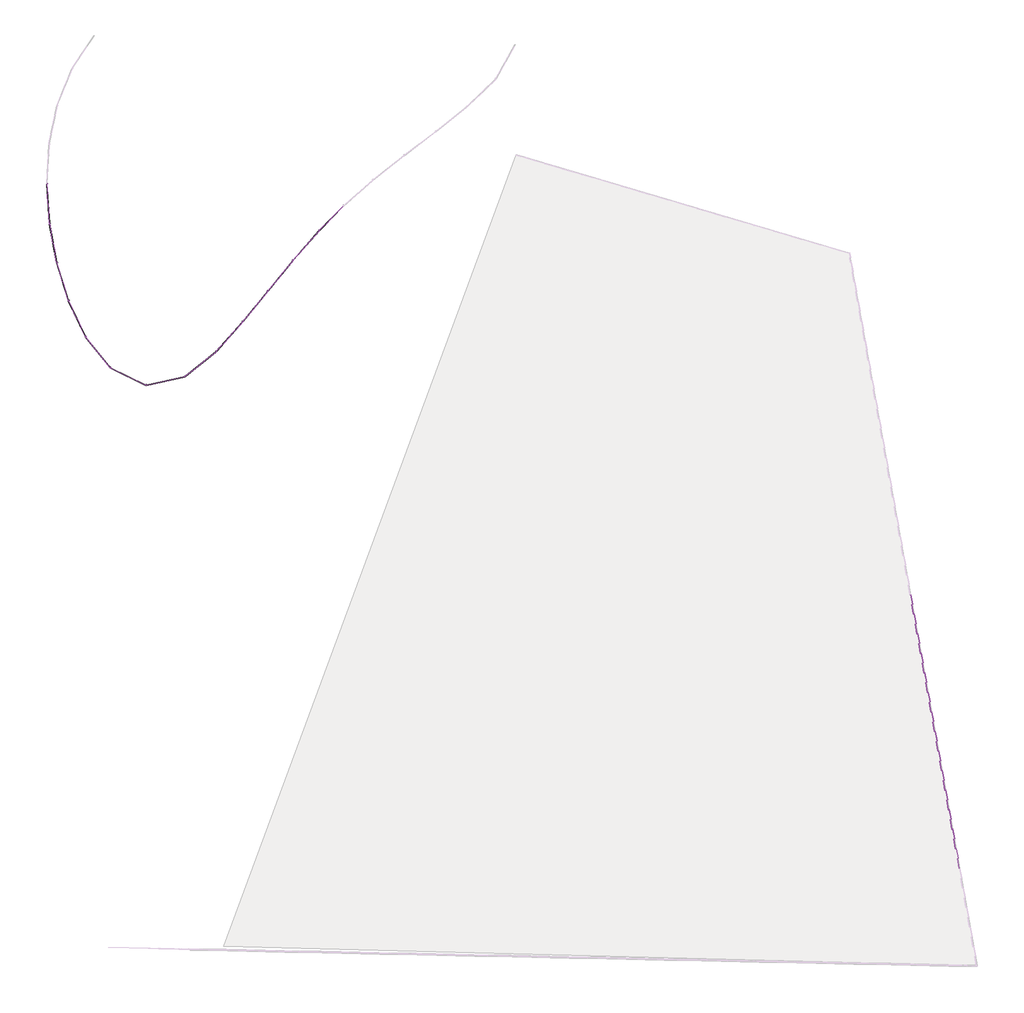
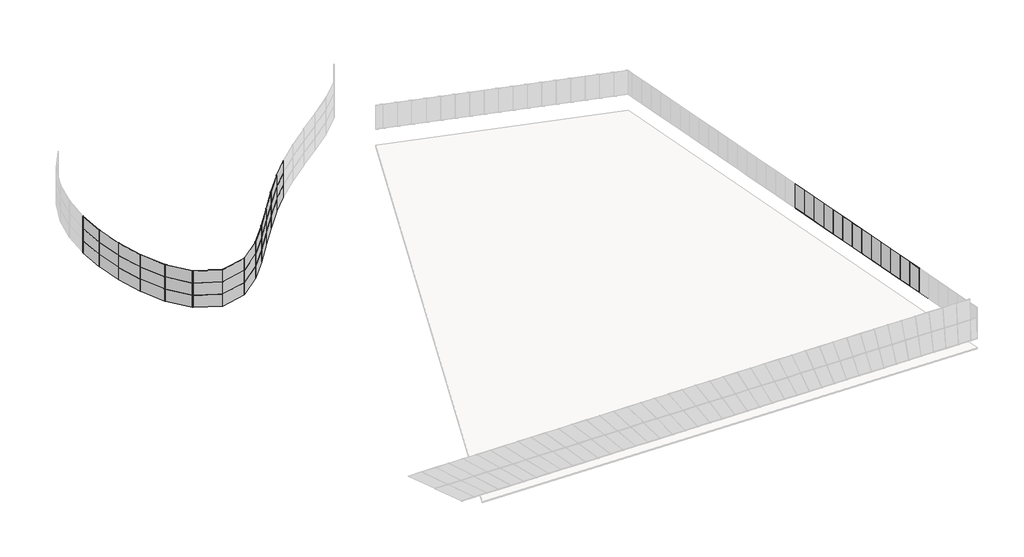
# One storey, part 3 of 5: 54 members, 52 plates.
"""IFC4 building model written with IfcOpenShell, lengths in millimetres."""

import ifcopenshell
import ifcopenshell.guid

model = None  # the IFC model being written
_history = None  # IfcOwnerHistory: only IFC2X3 demands one
_inside = {}  # id of a spatial element -> (the spatial element, [elements in it])
_under = {}  # id of a project, library or spatial element -> (it, [spatial elements below it])
_declared = {}  # id of a project -> (the project, [libraries it declares])
_typed = {}  # id of a type object -> (the type object, [elements of that type])
_made_of = {}  # id of a material, layer set ... -> (it, [elements and type objects made of it])


def new_model(schema):
    """Start an empty IFC model of exactly this schema.

    Asked for "IFC4X3", IfcOpenShell would pick the latest addendum, in which some entities
    have other attributes; the version numbers below select the first issue.
    IFC2X3 requires an IfcOwnerHistory on every rooted entity: one is made here for all.
    """
    global model, _history
    if schema == "IFC4X3":
        model = ifcopenshell.file(schema_version=(4, 3, 0, 0))
    else:
        model = ifcopenshell.file(schema=schema)
    _inside.clear()
    _under.clear()
    _declared.clear()
    _typed.clear()
    _made_of.clear()
    _history = None
    if model.schema == "IFC2X3":
        org = make("IfcOrganization", Name="unknown")
        user = make(
            "IfcPersonAndOrganization",
            ThePerson=make("IfcPerson", FamilyName="unknown"),
            TheOrganization=org,
        )
        app = make(
            "IfcApplication",
            ApplicationDeveloper=org,
            Version="unknown",
            ApplicationFullName="unknown",
            ApplicationIdentifier="unknown",
        )
        _history = make(
            "IfcOwnerHistory",
            OwningUser=user,
            OwningApplication=app,
            ChangeAction="ADDED",
            CreationDate=0,
        )
    return model


def make(cls, **values):
    """One entity of the class cls with the attributes given. An attribute that is None is left unset."""
    return model.create_entity(
        cls, **{name: value for name, value in values.items() if value is not None}
    )


def rooted(cls, **values):
    """An entity with a GlobalId (a new one), such as an element, a storey or a relation."""
    return make(cls, GlobalId=ifcopenshell.guid.new(), OwnerHistory=_history, **values)


def si_unit(unit_type, name, prefix=None):
    """IfcSIUnit, for example si_unit("LENGTHUNIT", "METRE", prefix="MILLI")."""
    return make("IfcSIUnit", UnitType=unit_type, Prefix=prefix, Name=name)


def assignment(units):
    """IfcUnitAssignment: the units of a project."""
    return None if units is None else make("IfcUnitAssignment", Units=units)


def point(xyz):
    """IfcCartesianPoint."""
    return None if xyz is None else make("IfcCartesianPoint", Coordinates=xyz)


def direction(xyz):
    """IfcDirection."""
    return None if xyz is None else make("IfcDirection", DirectionRatios=xyz)


def frame(location, z_axis=None, x_axis=None):
    """IfcAxis2Placement3D, a coordinate frame: its origin and axes. An axis left out is left unset."""
    return make(
        "IfcAxis2Placement3D",
        Location=point(location),
        Axis=direction(z_axis),
        RefDirection=direction(x_axis),
    )


def frame_2d(location, x_axis=None):
    """IfcAxis2Placement2D, a coordinate frame in the plane: its origin and x axis."""
    return make(
        "IfcAxis2Placement2D", Location=point(location), RefDirection=direction(x_axis)
    )


def origin():
    """The frame at (0, 0, 0) with its axes left unset."""
    return frame((0.0, 0.0, 0.0))


def origin_with_axes():
    """The frame at (0, 0, 0) with the z axis (0, 0, 1) and the x axis (1, 0, 0) written out."""
    return frame((0.0, 0.0, 0.0), z_axis=(0.0, 0.0, 1.0), x_axis=(1.0, 0.0, 0.0))


def origin_2d():
    """The frame at (0, 0) in the plane with its x axis left unset."""
    return frame_2d((0.0, 0.0))


def place(relative_to, where):
    """IfcLocalPlacement: puts the frame where relative to a parent placement (None: the world)."""
    return make(
        "IfcLocalPlacement", PlacementRelTo=relative_to, RelativePlacement=where
    )


def context(
    kind, dimensions, precision=None, world=None, true_north=None, identifier=None
):
    """IfcGeometricRepresentationContext, for example the 3D "Model" context."""
    return make(
        "IfcGeometricRepresentationContext",
        ContextIdentifier=identifier,
        ContextType=kind,
        CoordinateSpaceDimension=dimensions,
        Precision=precision,
        WorldCoordinateSystem=world,
        TrueNorth=true_north,
    )


def project(units=None, contexts=None):
    """IfcProject with its units and contexts."""
    return rooted(
        "IfcProject",
        Name="project",
        RepresentationContexts=contexts,
        UnitsInContext=assignment(units),
    )


def spatial(cls, under=None, at=None, **own):
    """A site, building, storey or space (cls), placed at a placement, below another one or the project."""
    s = rooted(cls, ObjectPlacement=at, **own)
    if under is not None:
        _under.setdefault(under.id(), (under, []))[1].append(s)
    return s


def polyline(points):
    """IfcPolyline through the points."""
    return make("IfcPolyline", Points=[point(p) for p in points])


def circle_curve(where, radius):
    """IfcCircle in the frame where."""
    return make("IfcCircle", Position=where, Radius=radius)


def trimmed(basis, trim1, trim2, sense, master):
    """IfcTrimmedCurve: the piece of a basis curve between two trims."""
    return make(
        "IfcTrimmedCurve",
        BasisCurve=basis,
        Trim1=trim1,
        Trim2=trim2,
        SenseAgreement=sense,
        MasterRepresentation=master,
    )


def segment(curve, same_sense, transition):
    """IfcCompositeCurveSegment."""
    return make(
        "IfcCompositeCurveSegment",
        Transition=transition,
        SameSense=same_sense,
        ParentCurve=curve,
    )


def composite_curve(segments, self_intersect=None):
    """IfcCompositeCurve: segments joined end to end."""
    return make("IfcCompositeCurve", Segments=segments, SelfIntersect=self_intersect)


def outline(outer, holes=None, kind="AREA"):
    """IfcArbitraryClosedProfileDef: a profile drawn as a closed curve; with holes, ...WithVoids."""
    if holes is None:
        return make("IfcArbitraryClosedProfileDef", ProfileType=kind, OuterCurve=outer)
    return make(
        "IfcArbitraryProfileDefWithVoids",
        ProfileType=kind,
        OuterCurve=outer,
        InnerCurves=holes,
    )


def extrude(swept, where, along, depth):
    """IfcExtrudedAreaSolid: the profile swept, set in the frame where, extruded along a direction by depth."""
    return make(
        "IfcExtrudedAreaSolid",
        SweptArea=swept,
        Position=where,
        ExtrudedDirection=direction(along),
        Depth=depth,
    )


def shape(context_of_items, identifier, shape_type, items):
    """IfcShapeRepresentation: the items that make up one representation, for example the "Body"."""
    return make(
        "IfcShapeRepresentation",
        ContextOfItems=context_of_items,
        RepresentationIdentifier=identifier,
        RepresentationType=shape_type,
        Items=items,
    )


def source(mapping_origin, context_of_items, identifier, shape_type, items):
    """IfcRepresentationMap: a shape defined once, which mapped items show again and again."""
    return make(
        "IfcRepresentationMap",
        MappingOrigin=mapping_origin,
        MappedRepresentation=shape(context_of_items, identifier, shape_type, items),
    )


def transform(
    local_origin,
    x_axis=None,
    y_axis=None,
    z_axis=None,
    scale=None,
    scale2=None,
    scale3=None,
    uniform=True,
):
    """IfcCartesianTransformationOperator3D, or its non-uniform kind. x_axis, y_axis, z_axis: its Axis1, 2, 3."""
    if uniform:
        return make(
            "IfcCartesianTransformationOperator3D",
            Axis1=direction(x_axis),
            Axis2=direction(y_axis),
            LocalOrigin=point(local_origin),
            Scale=scale,
            Axis3=direction(z_axis),
        )
    return make(
        "IfcCartesianTransformationOperator3DnonUniform",
        Axis1=direction(x_axis),
        Axis2=direction(y_axis),
        LocalOrigin=point(local_origin),
        Scale=scale,
        Axis3=direction(z_axis),
        Scale2=scale2,
        Scale3=scale3,
    )


def mapped(mapping_source, mapping_target):
    """IfcMappedItem: shows the shape of a source again, moved by a transform."""
    return make(
        "IfcMappedItem", MappingSource=mapping_source, MappingTarget=mapping_target
    )


def made_of(thing, what):
    """Note that an element or type object is made of a material, layer set ...; save() writes the relation."""
    if what is not None:
        _made_of.setdefault(what.id(), (what, []))[1].append(thing)
    return thing


def element(
    cls,
    number,
    at=None,
    inside=None,
    cuts=None,
    type_object=None,
    material=None,
    context=None,
    identifier="Body",
    shape_type=None,
    held_by="IfcProductDefinitionShape",
    body=None,
    shapes=None,
    **own,
):
    """One element of the class cls, such as IfcWall. Its Tag is "e" and its number.

    at: its placement. inside: the storey or other place that contains it. cuts: it is an
    opening in that element (IfcRelVoidsElement). A single representation is given by context,
    identifier, shape_type and body (its items); several are given by shapes. held_by: the class
    of the entity that holds the representations. save() writes the other relations.
    """
    e = rooted(cls, Tag="e%d" % number, ObjectPlacement=at, **own)
    if body is not None:
        shapes = [shape(context, identifier, shape_type, body)]
    if shapes is not None:
        e.Representation = make(held_by, Representations=shapes)
    if inside is not None:
        _inside.setdefault(inside.id(), (inside, []))[1].append(e)
    if cuts is not None:
        rooted(
            "IfcRelVoidsElement", RelatingBuildingElement=cuts, RelatedOpeningElement=e
        )
    if type_object is not None:
        _typed.setdefault(type_object.id(), (type_object, []))[1].append(e)
    return made_of(e, material)


def aggregate(whole, parts):
    """IfcRelAggregates: a whole, such as a stair, and the parts it consists of."""
    return rooted("IfcRelAggregates", RelatingObject=whole, RelatedObjects=parts)


def save(model, path):
    """Write the relations noted so far, then the file.

    IfcRelAggregates (storeys below a building ...), IfcRelContainedInSpatialStructure (elements
    in a storey), IfcRelDefinesByType, IfcRelAssociatesMaterial and IfcRelDeclares: one each for
    every whole, place, type object, material and project.
    """
    for whole, parts in _under.values():
        aggregate(whole, parts)
    for where, things in _inside.values():
        rooted(
            "IfcRelContainedInSpatialStructure",
            RelatedElements=things,
            RelatingStructure=where,
        )
    for kind, things in _typed.values():
        rooted("IfcRelDefinesByType", RelatedObjects=things, RelatingType=kind)
    for what, things in _made_of.values():
        rooted("IfcRelAssociatesMaterial", RelatedObjects=things, RelatingMaterial=what)
    for by, libraries in _declared.values():
        rooted("IfcRelDeclares", RelatingContext=by, RelatedDefinitions=libraries)
    model.write(path)


def montante_circular_25_mm_raio_36e581cf(model_context):
    return source(origin(), model_context, "Body", "SweptSolid", [
        extrude(outline(composite_curve([segment(trimmed(circle_curve(origin_2d(), 25.0), [point((25.0, 0.0))], [point((-25.0, 0.0))], False, "CARTESIAN"), True, "CONTINUOUS"), segment(trimmed(circle_curve(origin_2d(), 25.0), [point((-25.0, 0.0))], [point((25.0, 0.0))], False, "CARTESIAN"), True, "CONTINUOUS")], self_intersect=False)), frame((0.0, 0.0, -1500.0), z_axis=(0.0, 0.0, 1.0), x_axis=(1.0, 0.0, 0.0)), (0.0, 0.0, 1.0), 1500.0),
    ])


def montante_circular_25_mm_raio_ce826986(model_context):
    return source(origin(), model_context, "Body", "SweptSolid", [
        extrude(outline(composite_curve([segment(trimmed(circle_curve(frame_2d((-25.0, 0.0)), 25.0), [point((0.0, 0.0))], [point((-50.0, 0.0))], False, "CARTESIAN"), True, "CONTINUOUS"), segment(trimmed(circle_curve(frame_2d((-25.0, 0.0)), 25.0), [point((-50.0, 0.0))], [point((0.0, 0.0))], False, "CARTESIAN"), True, "CONTINUOUS")], self_intersect=False)), frame((0.0, 0.0, -1500.0), z_axis=(0.0, 0.0, 1.0), x_axis=(1.0, 0.0, 0.0)), (0.0, 0.0, 1.0), 1500.0),
    ])


def painel_do_sistema_5ef9eced(model_context):
    return source(origin(), model_context, "Body", "SweptSolid", [
        extrude(outline(polyline([(1475.0, 24.5), (-1475.0, 24.5), (-1475.0, 49.5), (1475.0, 49.5), (1475.0, 24.5)])), origin_with_axes(), (0.0, 0.0, 1.0), 1500.0),
    ])


def painel_do_sistema_85ccde5d(model_context):
    return source(origin(), model_context, "Body", "SweptSolid", [
        extrude(outline(polyline([(1475.0, -49.5), (-1475.0, -49.5), (-1475.0, -24.5), (1475.0, -24.5), (1475.0, -49.5)])), origin_with_axes(), (0.0, 0.0, 1.0), 1500.0),
    ])


def painel_do_sistema_bfc8fefc(model_context):
    return source(origin(), model_context, "Body", "SweptSolid", [
        extrude(outline(polyline([(1275.8375317, -49.5), (-1275.8375317, -49.5), (-1275.8375317, -24.5), (1275.8375317, -24.5), (1275.8375317, -49.5)])), origin_with_axes(), (0.0, 0.0, 1.0), 1500.0),
    ])


model = new_model("IFC4")

# Units and contexts
model_context = context("Model", 3, world=origin())
ifc_project = project(units=[si_unit("LENGTHUNIT", "METRE", prefix="MILLI")], contexts=[model_context])

# Site, building, storey
site = spatial("IfcSite", under=ifc_project)
building = spatial("IfcBuilding", under=site)
storey = spatial("IfcBuildingStorey", under=building, Name="Nível 2", Elevation=4000.0)

# Members
placement = place(None, origin())
montante_circular_25_mm_raio_shape = montante_circular_25_mm_raio_36e581cf(model_context)
element("IfcMember", 1, ObjectType="Montante circular : 25 mm Raio", at=placement, inside=storey, context=model_context, shape_type="MappedRepresentation", body=[
    mapped(montante_circular_25_mm_raio_shape, transform((26678.2388316, -19401.0862995, 6000.000015), x_axis=(0.0, 0.0, 1.0), y_axis=(0.9843520034862617, 0.17621331740984483, 0.0), z_axis=(-0.1762133174098448, 0.9843520034862616, 0.0))),
])
element("IfcMember", 2, ObjectType="Montante circular : 25 mm Raio", at=placement, inside=storey, context=model_context, shape_type="MappedRepresentation", body=[
    mapped(montante_circular_25_mm_raio_shape, transform((26413.9188555, -17924.5582943, 6000.000015), x_axis=(0.0, 0.0, 1.0), y_axis=(0.9843520034862608, 0.1762133174098499, 0.0), z_axis=(-0.17621331740984988, 0.9843520034862606, 0.0))),
])
element("IfcMember", 3, ObjectType="Montante circular : 25 mm Raio", at=placement, inside=storey, context=model_context, shape_type="MappedRepresentation", body=[
    mapped(montante_circular_25_mm_raio_shape, transform((26149.5988794, -16448.030289, 6000.000015), x_axis=(0.0, 0.0, 1.0), y_axis=(0.9843520034862608, 0.1762133174098494, 0.0), z_axis=(-0.1762133174098494, 0.9843520034862608, 0.0))),
])
element("IfcMember", 4, ObjectType="Montante circular : 25 mm Raio", at=placement, inside=storey, context=model_context, shape_type="MappedRepresentation", body=[
    mapped(montante_circular_25_mm_raio_shape, transform((25885.2789032, -14971.5022838, 6000.000015), x_axis=(0.0, 0.0, 1.0), y_axis=(0.9843520034862613, 0.1762133174098471, 0.0), z_axis=(-0.17621331740984708, 0.9843520034862612, 0.0))),
])
element("IfcMember", 5, ObjectType="Montante circular : 25 mm Raio", at=placement, inside=storey, context=model_context, shape_type="MappedRepresentation", body=[
    mapped(montante_circular_25_mm_raio_shape, transform((25620.9589271, -13494.9742786, 6000.000015), x_axis=(0.0, 0.0, 1.0), y_axis=(0.9843520034862614, 0.1762133174098466, 0.0), z_axis=(-0.1762133174098466, 0.9843520034862614, 0.0))),
])
element("IfcMember", 6, ObjectType="Montante circular : 25 mm Raio", at=placement, inside=storey, context=model_context, shape_type="MappedRepresentation", body=[
    mapped(montante_circular_25_mm_raio_shape, transform((25356.638951, -12018.4462733, 6000.000015), x_axis=(0.0, 0.0, 1.0), y_axis=(0.9843520034862608, 0.17621331740984966, 0.0), z_axis=(-0.17621331740984966, 0.9843520034862608, 0.0))),
])
element("IfcMember", 7, ObjectType="Montante circular : 25 mm Raio", at=placement, inside=storey, context=model_context, shape_type="MappedRepresentation", body=[
    mapped(montante_circular_25_mm_raio_shape, transform((25092.3189749, -10541.9182681, 6000.000015), x_axis=(0.0, 0.0, 1.0), y_axis=(0.9843520034862613, 0.1762133174098471, 0.0), z_axis=(-0.17621331740984708, 0.9843520034862612, 0.0))),
])
element("IfcMember", 8, ObjectType="Montante circular : 25 mm Raio", at=placement, inside=storey, context=model_context, shape_type="MappedRepresentation", body=[
    mapped(montante_circular_25_mm_raio_shape, transform((24827.9989988, -9065.3902629, 6000.000015), x_axis=(0.0, 0.0, 1.0), y_axis=(0.9843520034862608, 0.1762133174098499, 0.0), z_axis=(-0.17621331740984988, 0.9843520034862606, 0.0))),
])
element("IfcMember", 9, ObjectType="Montante circular : 25 mm Raio", at=placement, inside=storey, context=model_context, shape_type="MappedRepresentation", body=[
    mapped(montante_circular_25_mm_raio_shape, transform((24563.6790227, -7588.8622577, 6000.000015), x_axis=(0.0, 0.0, 1.0), y_axis=(0.9843520034862613, 0.17621331740984686, 0.0), z_axis=(-0.17621331740984683, 0.9843520034862612, 0.0))),
])
element("IfcMember", 10, ObjectType="Montante circular : 25 mm Raio", at=placement, inside=storey, context=model_context, shape_type="MappedRepresentation", body=[
    mapped(montante_circular_25_mm_raio_shape, transform((24299.3590466, -6112.3342524, 6000.000015), x_axis=(0.0, 0.0, 1.0), y_axis=(0.9843520034862608, 0.17621331740984966, 0.0), z_axis=(-0.17621331740984966, 0.9843520034862608, 0.0))),
])
element("IfcMember", 11, ObjectType="Montante circular : 25 mm Raio", at=placement, inside=storey, context=model_context, shape_type="MappedRepresentation", body=[
    mapped(montante_circular_25_mm_raio_shape, transform((24035.0390704, -4635.8062472, 6000.000015), x_axis=(0.0, 0.0, 1.0), y_axis=(0.9843520034862608, 0.1762133174098499, 0.0), z_axis=(-0.17621331740984988, 0.9843520034862606, 0.0))),
])
element("IfcMember", 12, ObjectType="Montante circular : 25 mm Raio", at=placement, inside=storey, context=model_context, shape_type="MappedRepresentation", body=[
    mapped(montante_circular_25_mm_raio_shape, transform((23770.7190943, -3159.278242, 6000.000015), x_axis=(0.0, 0.0, 1.0), y_axis=(0.9843520034862614, 0.1762133174098466, 0.0), z_axis=(-0.1762133174098466, 0.9843520034862614, 0.0))),
])
element("IfcMember", 13, ObjectType="Montante circular : 25 mm Raio", at=placement, inside=storey, context=model_context, shape_type="MappedRepresentation", body=[
    mapped(montante_circular_25_mm_raio_shape, transform((23506.3991182, -1682.7502367, 6000.000015), x_axis=(0.0, 0.0, 1.0), y_axis=(0.9843520034862614, 0.17621331740984658, 0.0), z_axis=(-0.17621331740984655, 0.9843520034862612, 0.0))),
])
element("IfcMember", 14, ObjectType="Montante circular : 25 mm Raio", at=placement, inside=storey, context=model_context, shape_type="MappedRepresentation", body=[
    mapped(montante_circular_25_mm_raio_shape, transform((23242.0791421, -206.2222315, 6000.000015), x_axis=(0.0, 0.0, 1.0), y_axis=(0.9843520034862611, 0.17621331740984805, 0.0), z_axis=(-0.17621331740984805, 0.9843520034862611, 0.0))),
])
element("IfcMember", 15, ObjectType="Montante circular : 25 mm Raio", at=placement, inside=storey, context=model_context, shape_type="MappedRepresentation", body=[
    mapped(montante_circular_25_mm_raio_shape, transform((-41927.7364355, 30807.566003, 4500.0), x_axis=(0.00926833746122375, -0.999957048037917, 0.0), y_axis=(-0.999957048037917, -0.00926833746122375, 0.0), z_axis=(0.0, 0.0, -1.0))),
])
element("IfcMember", 16, ObjectType="Montante circular : 25 mm Raio", at=placement, inside=storey, context=model_context, shape_type="MappedRepresentation", body=[
    mapped(montante_circular_25_mm_raio_shape, transform((-41719.5366875, 27814.7992454, 4500.0), x_axis=(0.12720739477424994, -0.9918761408133316, 0.0), y_axis=(-0.9918761408133316, -0.12720739477424994, 0.0), z_axis=(0.0, 0.0, -1.0))),
])
element("IfcMember", 17, ObjectType="Montante circular : 25 mm Raio", at=placement, inside=storey, context=model_context, shape_type="MappedRepresentation", body=[
    mapped(montante_circular_25_mm_raio_shape, transform((-41172.4912602, 24865.0973452, 4500.0), x_axis=(0.23687893376105146, -0.9715391761222125, 0.0), y_axis=(-0.9715391761222125, -0.23687893376105146, 0.0), z_axis=(0.0, 0.0, -1.0))),
])
element("IfcMember", 18, ObjectType="Montante circular : 25 mm Raio", at=placement, inside=storey, context=model_context, shape_type="MappedRepresentation", body=[
    mapped(montante_circular_25_mm_raio_shape, transform((-40291.7668402, 21997.2890363, 4500.0), x_axis=(0.35274082804666734, -0.9357210632602814, 0.0), y_axis=(-0.9357210632602814, -0.35274082804666734, 0.0), z_axis=(0.0, 0.0, -1.0))),
])
element("IfcMember", 19, ObjectType="Montante circular : 25 mm Raio", at=placement, inside=storey, context=model_context, shape_type="MappedRepresentation", body=[
    mapped(montante_circular_25_mm_raio_shape, transform((-39014.8508906, 19282.6093761, 4500.0), x_axis=(0.5079873162147126, -0.8613645491689182, 0.0), y_axis=(-0.8613645491689182, -0.5079873162147126, 0.0), z_axis=(0.0, 0.0, -1.0))),
])
element("IfcMember", 20, ObjectType="Montante circular : 25 mm Raio", at=placement, inside=storey, context=model_context, shape_type="MappedRepresentation", body=[
    mapped(montante_circular_25_mm_raio_shape, transform((-37150.2365801, 16932.4575783, 4500.0), x_axis=(0.7466685294931728, -0.6651962921307538, 0.0), y_axis=(-0.6651962921307538, -0.7466685294931728, 0.0), z_axis=(0.0, 0.0, -1.0))),
])
element("IfcMember", 21, ObjectType="Montante circular : 25 mm Raio", at=placement, inside=storey, context=model_context, shape_type="MappedRepresentation", body=[
    mapped(montante_circular_25_mm_raio_shape, transform((-34451.4946749, 15622.1934334, 4500.0), x_axis=(0.9926557018483062, -0.12097378884719918, 0.0), y_axis=(-0.12097378884719918, -0.9926557018483062, 0.0), z_axis=(0.0, 0.0, -1.0))),
])
element("IfcMember", 22, ObjectType="Montante circular : 25 mm Raio", at=placement, inside=storey, context=model_context, shape_type="MappedRepresentation", body=[
    mapped(montante_circular_25_mm_raio_shape, transform((-31525.1733328, 16282.9834173, 4500.0), x_axis=(0.870163483817595, 0.49276313927730647, 0.0), y_axis=(0.49276313927730647, -0.870163483817595, 0.0), z_axis=(0.0, 0.0, -1.0))),
])
element("IfcMember", 23, ObjectType="Montante circular : 25 mm Raio", at=placement, inside=storey, context=model_context, shape_type="MappedRepresentation", body=[
    mapped(montante_circular_25_mm_raio_shape, transform((-29189.3459235, 18165.5110569, 4500.0), x_axis=(0.7046961293095542, 0.7095092426009207, 0.0), y_axis=(0.7095092426009207, -0.7046961293095542, 0.0), z_axis=(0.0, 0.0, -1.0))),
])
element("IfcMember", 24, ObjectType="Montante circular : 25 mm Raio", at=placement, inside=storey, context=model_context, shape_type="MappedRepresentation", body=[
    mapped(montante_circular_25_mm_raio_shape, transform((-27187.2576877, 20399.7095029, 4500.0), x_axis=(0.6410206876840713, 0.7675236009146822, 0.0), y_axis=(0.7675236009146822, -0.6410206876840713, 0.0), z_axis=(0.0, 0.0, -1.0))),
])
element("IfcMember", 25, ObjectType="Montante circular : 25 mm Raio", at=placement, inside=storey, context=model_context, shape_type="MappedRepresentation", body=[
    mapped(montante_circular_25_mm_raio_shape, transform((-25293.7553869, 22726.6493467, 4500.0), x_axis=(0.6272671926241683, 0.7788041275297625, 0.0), y_axis=(0.7788041275297625, -0.6272671926241683, 0.0), z_axis=(0.0, 0.0, -1.0))),
])
element("IfcMember", 26, ObjectType="Montante circular : 25 mm Raio", at=placement, inside=storey, context=model_context, shape_type="MappedRepresentation", body=[
    mapped(montante_circular_25_mm_raio_shape, transform((-23394.8086307, 25049.1482632, 4500.0), x_axis=(0.6426798456549805, 0.766134854962813, 0.0), y_axis=(0.766134854962813, -0.6426798456549805, 0.0), z_axis=(0.0, 0.0, -1.0))),
])
element("IfcMember", 27, ObjectType="Montante circular : 25 mm Raio", at=placement, inside=storey, context=model_context, shape_type="MappedRepresentation", body=[
    mapped(montante_circular_25_mm_raio_shape, transform((-21416.0981725, 27304.0772915, 4500.0), x_axis=(0.6795654424505699, 0.7336148917701719, 0.0), y_axis=(0.7336148917701719, -0.6795654424505699, 0.0), z_axis=(0.0, 0.0, -1.0))),
])
element("IfcMember", 28, ObjectType="Montante circular : 25 mm Raio", at=placement, inside=storey, context=model_context, shape_type="MappedRepresentation", body=[
    mapped(montante_circular_25_mm_raio_shape, transform((-41927.7364355, 30807.566003, 6000.0), x_axis=(0.009268337461223849, -0.999957048037917, 0.0), y_axis=(-0.999957048037917, -0.009268337461223849, 0.0), z_axis=(0.0, 0.0, -1.0))),
])
element("IfcMember", 29, ObjectType="Montante circular : 25 mm Raio", at=placement, inside=storey, context=model_context, shape_type="MappedRepresentation", body=[
    mapped(montante_circular_25_mm_raio_shape, transform((-41719.5366875, 27814.7992454, 6000.0), x_axis=(0.12720739477424994, -0.9918761408133316, 0.0), y_axis=(-0.9918761408133316, -0.12720739477424994, 0.0), z_axis=(0.0, 0.0, -1.0))),
])
element("IfcMember", 30, ObjectType="Montante circular : 25 mm Raio", at=placement, inside=storey, context=model_context, shape_type="MappedRepresentation", body=[
    mapped(montante_circular_25_mm_raio_shape, transform((-41172.4912602, 24865.0973452, 6000.0), x_axis=(0.23687893376105146, -0.9715391761222125, 0.0), y_axis=(-0.9715391761222125, -0.23687893376105146, 0.0), z_axis=(0.0, 0.0, -1.0))),
])
element("IfcMember", 31, ObjectType="Montante circular : 25 mm Raio", at=placement, inside=storey, context=model_context, shape_type="MappedRepresentation", body=[
    mapped(montante_circular_25_mm_raio_shape, transform((-40291.7668402, 21997.2890363, 6000.0), x_axis=(0.35274082804666723, -0.9357210632602814, 0.0), y_axis=(-0.9357210632602814, -0.35274082804666723, 0.0), z_axis=(0.0, 0.0, -1.0))),
])
element("IfcMember", 32, ObjectType="Montante circular : 25 mm Raio", at=placement, inside=storey, context=model_context, shape_type="MappedRepresentation", body=[
    mapped(montante_circular_25_mm_raio_shape, transform((-39014.8508906, 19282.6093761, 6000.0), x_axis=(0.5079873162147126, -0.8613645491689182, 0.0), y_axis=(-0.8613645491689182, -0.5079873162147126, 0.0), z_axis=(0.0, 0.0, -1.0))),
])
element("IfcMember", 33, ObjectType="Montante circular : 25 mm Raio", at=placement, inside=storey, context=model_context, shape_type="MappedRepresentation", body=[
    mapped(montante_circular_25_mm_raio_shape, transform((-37150.2365801, 16932.4575783, 6000.0), x_axis=(0.7466685294931725, -0.665196292130754, 0.0), y_axis=(-0.665196292130754, -0.7466685294931725, 0.0), z_axis=(0.0, 0.0, -1.0))),
])
element("IfcMember", 34, ObjectType="Montante circular : 25 mm Raio", at=placement, inside=storey, context=model_context, shape_type="MappedRepresentation", body=[
    mapped(montante_circular_25_mm_raio_shape, transform((-34451.4946749, 15622.1934334, 6000.0), x_axis=(0.9926557018483062, -0.12097378884719918, 0.0), y_axis=(-0.12097378884719918, -0.9926557018483062, 0.0), z_axis=(0.0, 0.0, -1.0))),
])
element("IfcMember", 35, ObjectType="Montante circular : 25 mm Raio", at=placement, inside=storey, context=model_context, shape_type="MappedRepresentation", body=[
    mapped(montante_circular_25_mm_raio_shape, transform((-31525.1733328, 16282.9834173, 6000.0), x_axis=(0.870163483817595, 0.49276313927730647, 0.0), y_axis=(0.49276313927730647, -0.870163483817595, 0.0), z_axis=(0.0, 0.0, -1.0))),
])
element("IfcMember", 36, ObjectType="Montante circular : 25 mm Raio", at=placement, inside=storey, context=model_context, shape_type="MappedRepresentation", body=[
    mapped(montante_circular_25_mm_raio_shape, transform((-29189.3459235, 18165.5110569, 6000.0), x_axis=(0.7046961293095542, 0.7095092426009207, 0.0), y_axis=(0.7095092426009207, -0.7046961293095542, 0.0), z_axis=(0.0, 0.0, -1.0))),
])
element("IfcMember", 37, ObjectType="Montante circular : 25 mm Raio", at=placement, inside=storey, context=model_context, shape_type="MappedRepresentation", body=[
    mapped(montante_circular_25_mm_raio_shape, transform((-27187.2576877, 20399.7095029, 6000.0), x_axis=(0.6410206876840709, 0.7675236009146824, 0.0), y_axis=(0.7675236009146824, -0.6410206876840709, 0.0), z_axis=(0.0, 0.0, -1.0))),
])
element("IfcMember", 38, ObjectType="Montante circular : 25 mm Raio", at=placement, inside=storey, context=model_context, shape_type="MappedRepresentation", body=[
    mapped(montante_circular_25_mm_raio_shape, transform((-25293.7553869, 22726.6493467, 6000.0), x_axis=(0.627267192624168, 0.7788041275297628, 0.0), y_axis=(0.7788041275297628, -0.627267192624168, 0.0), z_axis=(0.0, 0.0, -1.0))),
])
element("IfcMember", 39, ObjectType="Montante circular : 25 mm Raio", at=placement, inside=storey, context=model_context, shape_type="MappedRepresentation", body=[
    mapped(montante_circular_25_mm_raio_shape, transform((-23394.8086307, 25049.1482632, 6000.0), x_axis=(0.6426798456549805, 0.7661348549628131, 0.0), y_axis=(0.7661348549628131, -0.6426798456549805, 0.0), z_axis=(0.0, 0.0, -1.0))),
])
element("IfcMember", 40, ObjectType="Montante circular : 25 mm Raio", at=placement, inside=storey, context=model_context, shape_type="MappedRepresentation", body=[
    mapped(montante_circular_25_mm_raio_shape, transform((-21416.0981725, 27304.0772915, 6000.0), x_axis=(0.6795654424505698, 0.7336148917701721, 0.0), y_axis=(0.7336148917701721, -0.6795654424505698, 0.0), z_axis=(0.0, 0.0, -1.0))),
])
element("IfcMember", 41, ObjectType="Montante circular : 25 mm Raio", at=placement, inside=storey, context=model_context, shape_type="MappedRepresentation", body=[
    mapped(montante_circular_25_mm_raio_shape, transform((-41927.7364355, 30807.566003, 7500.0), x_axis=(0.00926833746122375, -0.999957048037917, 0.0), y_axis=(-0.999957048037917, -0.00926833746122375, 0.0), z_axis=(0.0, 0.0, -1.0))),
])
element("IfcMember", 42, ObjectType="Montante circular : 25 mm Raio", at=placement, inside=storey, context=model_context, shape_type="MappedRepresentation", body=[
    mapped(montante_circular_25_mm_raio_shape, transform((-41719.5366875, 27814.7992454, 7500.0), x_axis=(0.12720739477424994, -0.9918761408133316, 0.0), y_axis=(-0.9918761408133316, -0.12720739477424994, 0.0), z_axis=(0.0, 0.0, -1.0))),
])
element("IfcMember", 43, ObjectType="Montante circular : 25 mm Raio", at=placement, inside=storey, context=model_context, shape_type="MappedRepresentation", body=[
    mapped(montante_circular_25_mm_raio_shape, transform((-41172.4912602, 24865.0973452, 7500.0), x_axis=(0.23687893376105146, -0.9715391761222125, 0.0), y_axis=(-0.9715391761222125, -0.23687893376105146, 0.0), z_axis=(0.0, 0.0, -1.0))),
])
element("IfcMember", 44, ObjectType="Montante circular : 25 mm Raio", at=placement, inside=storey, context=model_context, shape_type="MappedRepresentation", body=[
    mapped(montante_circular_25_mm_raio_shape, transform((-40291.7668402, 21997.2890363, 7500.0), x_axis=(0.3527408280466673, -0.9357210632602814, 0.0), y_axis=(-0.9357210632602814, -0.3527408280466673, 0.0), z_axis=(0.0, 0.0, -1.0))),
])
element("IfcMember", 45, ObjectType="Montante circular : 25 mm Raio", at=placement, inside=storey, context=model_context, shape_type="MappedRepresentation", body=[
    mapped(montante_circular_25_mm_raio_shape, transform((-39014.8508906, 19282.6093761, 7500.0), x_axis=(0.5079873162147126, -0.8613645491689182, 0.0), y_axis=(-0.8613645491689182, -0.5079873162147126, 0.0), z_axis=(0.0, 0.0, -1.0))),
])
element("IfcMember", 46, ObjectType="Montante circular : 25 mm Raio", at=placement, inside=storey, context=model_context, shape_type="MappedRepresentation", body=[
    mapped(montante_circular_25_mm_raio_shape, transform((-37150.2365801, 16932.4575783, 7500.0), x_axis=(0.7466685294931724, -0.665196292130754, 0.0), y_axis=(-0.665196292130754, -0.7466685294931724, 0.0), z_axis=(0.0, 0.0, -1.0))),
])
element("IfcMember", 47, ObjectType="Montante circular : 25 mm Raio", at=placement, inside=storey, context=model_context, shape_type="MappedRepresentation", body=[
    mapped(montante_circular_25_mm_raio_shape, transform((-34451.4946749, 15622.1934334, 7500.0), x_axis=(0.992655701848306, -0.12097378884720081, 0.0), y_axis=(-0.12097378884720081, -0.992655701848306, 0.0), z_axis=(0.0, 0.0, -1.0))),
])
element("IfcMember", 48, ObjectType="Montante circular : 25 mm Raio", at=placement, inside=storey, context=model_context, shape_type="MappedRepresentation", body=[
    mapped(montante_circular_25_mm_raio_shape, transform((-31525.1733328, 16282.9834173, 7500.0), x_axis=(0.870163483817595, 0.49276313927730647, 0.0), y_axis=(0.49276313927730647, -0.870163483817595, 0.0), z_axis=(0.0, 0.0, -1.0))),
])
element("IfcMember", 49, ObjectType="Montante circular : 25 mm Raio", at=placement, inside=storey, context=model_context, shape_type="MappedRepresentation", body=[
    mapped(montante_circular_25_mm_raio_shape, transform((-29189.3459235, 18165.5110569, 7500.0), x_axis=(0.7046961293095542, 0.7095092426009207, 0.0), y_axis=(0.7095092426009207, -0.7046961293095542, 0.0), z_axis=(0.0, 0.0, -1.0))),
])
element("IfcMember", 50, ObjectType="Montante circular : 25 mm Raio", at=placement, inside=storey, context=model_context, shape_type="MappedRepresentation", body=[
    mapped(montante_circular_25_mm_raio_shape, transform((-27187.2576877, 20399.7095029, 7500.0), x_axis=(0.6410206876840713, 0.7675236009146822, 0.0), y_axis=(0.7675236009146822, -0.6410206876840713, 0.0), z_axis=(0.0, 0.0, -1.0))),
])
element("IfcMember", 51, ObjectType="Montante circular : 25 mm Raio", at=placement, inside=storey, context=model_context, shape_type="MappedRepresentation", body=[
    mapped(montante_circular_25_mm_raio_shape, transform((-25293.7553869, 22726.6493467, 7500.0), x_axis=(0.627267192624168, 0.7788041275297628, 0.0), y_axis=(0.7788041275297628, -0.627267192624168, 0.0), z_axis=(0.0, 0.0, -1.0))),
])
element("IfcMember", 52, ObjectType="Montante circular : 25 mm Raio", at=placement, inside=storey, context=model_context, shape_type="MappedRepresentation", body=[
    mapped(montante_circular_25_mm_raio_shape, transform((-23394.8086307, 25049.1482632, 7500.0), x_axis=(0.6426798456549805, 0.7661348549628131, 0.0), y_axis=(0.7661348549628131, -0.6426798456549805, 0.0), z_axis=(0.0, 0.0, -1.0))),
])
element("IfcMember", 53, ObjectType="Montante circular : 25 mm Raio", at=placement, inside=storey, context=model_context, shape_type="MappedRepresentation", body=[
    mapped(montante_circular_25_mm_raio_shape, transform((-21416.0981725, 27304.0772915, 7500.0), x_axis=(0.6795654424505699, 0.7336148917701719, 0.0), y_axis=(0.7336148917701719, -0.6795654424505699, 0.0), z_axis=(0.0, 0.0, -1.0))),
])
montante_circular_25_mm_raio_2_shape = montante_circular_25_mm_raio_ce826986(model_context)
element("IfcMember", 54, ObjectType="Montante circular : 25 mm Raio", at=placement, inside=storey, context=model_context, shape_type="MappedRepresentation", body=[
    mapped(montante_circular_25_mm_raio_2_shape, transform((-19607.9031675, 29139.747525, 6000.0), x_axis=(-0.7515265818306623, -0.6597028094543185, 0.0), y_axis=(0.6597028094543185, -0.7515265818306623, 0.0), z_axis=(0.0, 0.0, 1.0))),
])

# Plates
painel_do_sistema_shape = painel_do_sistema_5ef9eced(model_context)
element("IfcPlate", 55, ObjectType="Painel do sistema : Envidraçado", at=placement, inside=storey, context=model_context, shape_type="MappedRepresentation", body=[
    mapped(painel_do_sistema_shape, transform((26413.9188555, -17924.5582943, 7500.00001), x_axis=(0.0, 0.0, 1.0), y_axis=(-0.9843520034862613, -0.1762133174098471, 0.0), z_axis=(0.1762133174098471, -0.9843520034862613, 0.0))),
])
element("IfcPlate", 56, ObjectType="Painel do sistema : Envidraçado", at=placement, inside=storey, context=model_context, shape_type="MappedRepresentation", body=[
    mapped(painel_do_sistema_shape, transform((26149.5988794, -16448.030289, 7500.00001), x_axis=(0.0, 0.0, 1.0), y_axis=(-0.9843520034862608, -0.1762133174098494, 0.0), z_axis=(0.1762133174098494, -0.9843520034862608, 0.0))),
])
element("IfcPlate", 57, ObjectType="Painel do sistema : Envidraçado", at=placement, inside=storey, context=model_context, shape_type="MappedRepresentation", body=[
    mapped(painel_do_sistema_shape, transform((25885.2789032, -14971.5022838, 7500.00001), x_axis=(0.0, 0.0, 1.0), y_axis=(-0.9843520034862613, -0.1762133174098471, 0.0), z_axis=(0.1762133174098471, -0.9843520034862613, 0.0))),
])
element("IfcPlate", 58, ObjectType="Painel do sistema : Envidraçado", at=placement, inside=storey, context=model_context, shape_type="MappedRepresentation", body=[
    mapped(painel_do_sistema_shape, transform((25620.9589271, -13494.9742786, 7500.00001), x_axis=(0.0, 0.0, 1.0), y_axis=(-0.9843520034862614, -0.1762133174098466, 0.0), z_axis=(0.1762133174098466, -0.9843520034862614, 0.0))),
])
element("IfcPlate", 59, ObjectType="Painel do sistema : Envidraçado", at=placement, inside=storey, context=model_context, shape_type="MappedRepresentation", body=[
    mapped(painel_do_sistema_shape, transform((25356.638951, -12018.4462733, 7500.00001), x_axis=(0.0, 0.0, 1.0), y_axis=(-0.9843520034862608, -0.17621331740984966, 0.0), z_axis=(0.17621331740984966, -0.9843520034862608, 0.0))),
])
element("IfcPlate", 60, ObjectType="Painel do sistema : Envidraçado", at=placement, inside=storey, context=model_context, shape_type="MappedRepresentation", body=[
    mapped(painel_do_sistema_shape, transform((25092.3189749, -10541.9182681, 7500.00001), x_axis=(0.0, 0.0, 1.0), y_axis=(-0.9843520034862608, -0.1762133174098499, 0.0), z_axis=(0.1762133174098499, -0.9843520034862608, 0.0))),
])
element("IfcPlate", 61, ObjectType="Painel do sistema : Envidraçado", at=placement, inside=storey, context=model_context, shape_type="MappedRepresentation", body=[
    mapped(painel_do_sistema_shape, transform((24827.9989988, -9065.3902629, 7500.00001), x_axis=(0.0, 0.0, 1.0), y_axis=(-0.9843520034862613, -0.1762133174098471, 0.0), z_axis=(0.1762133174098471, -0.9843520034862613, 0.0))),
])
element("IfcPlate", 62, ObjectType="Painel do sistema : Envidraçado", at=placement, inside=storey, context=model_context, shape_type="MappedRepresentation", body=[
    mapped(painel_do_sistema_shape, transform((24563.6790227, -7588.8622577, 7500.00001), x_axis=(0.0, 0.0, 1.0), y_axis=(-0.9843520034862608, -0.17621331740984966, 0.0), z_axis=(0.17621331740984966, -0.9843520034862608, 0.0))),
])
element("IfcPlate", 63, ObjectType="Painel do sistema : Envidraçado", at=placement, inside=storey, context=model_context, shape_type="MappedRepresentation", body=[
    mapped(painel_do_sistema_shape, transform((24299.3590466, -6112.3342524, 7500.00001), x_axis=(0.0, 0.0, 1.0), y_axis=(-0.9843520034862613, -0.17621331740984683, 0.0), z_axis=(0.17621331740984683, -0.9843520034862613, 0.0))),
])
element("IfcPlate", 64, ObjectType="Painel do sistema : Envidraçado", at=placement, inside=storey, context=model_context, shape_type="MappedRepresentation", body=[
    mapped(painel_do_sistema_shape, transform((24035.0390704, -4635.8062472, 7500.00001), x_axis=(0.0, 0.0, 1.0), y_axis=(-0.9843520034862608, -0.1762133174098499, 0.0), z_axis=(0.1762133174098499, -0.9843520034862608, 0.0))),
])
element("IfcPlate", 65, ObjectType="Painel do sistema : Envidraçado", at=placement, inside=storey, context=model_context, shape_type="MappedRepresentation", body=[
    mapped(painel_do_sistema_shape, transform((23770.7190943, -3159.278242, 7500.00001), x_axis=(0.0, 0.0, 1.0), y_axis=(-0.9843520034862614, -0.1762133174098466, 0.0), z_axis=(0.1762133174098466, -0.9843520034862614, 0.0))),
])
element("IfcPlate", 66, ObjectType="Painel do sistema : Envidraçado", at=placement, inside=storey, context=model_context, shape_type="MappedRepresentation", body=[
    mapped(painel_do_sistema_shape, transform((23506.3991182, -1682.7502367, 7500.00001), x_axis=(0.0, 0.0, 1.0), y_axis=(-0.9843520034862608, -0.1762133174098494, 0.0), z_axis=(0.1762133174098494, -0.9843520034862608, 0.0))),
])
element("IfcPlate", 67, ObjectType="Painel do sistema : Envidraçado", at=placement, inside=storey, context=model_context, shape_type="MappedRepresentation", body=[
    mapped(painel_do_sistema_shape, transform((23242.0791421, -206.2222315, 7500.00001), x_axis=(0.0, 0.0, 1.0), y_axis=(-0.9843520034862612, -0.1762133174098481, 0.0), z_axis=(0.1762133174098481, -0.9843520034862612, 0.0))),
])
painel_do_sistema_2_shape = painel_do_sistema_85ccde5d(model_context)
element("IfcPlate", 68, ObjectType="Painel do sistema : Envidraçado", at=placement, inside=storey, context=model_context, shape_type="MappedRepresentation", body=[
    mapped(painel_do_sistema_2_shape, transform((-41823.6365615, 29311.1826242, 4500.0), x_axis=(0.06939991602576077, -0.9975889191724302, 0.0), y_axis=(0.9975889191724302, 0.06939991602576077, 0.0), z_axis=(0.0, 0.0, 1.0))),
])
element("IfcPlate", 69, ObjectType="Painel do sistema : Envidraçado", at=placement, inside=storey, context=model_context, shape_type="MappedRepresentation", body=[
    mapped(painel_do_sistema_2_shape, transform((-41446.0139738, 26339.9482953, 4500.0), x_axis=(0.18234847575688512, -0.9832339667592555, 0.0), y_axis=(0.9832339667592555, 0.18234847575688512, 0.0), z_axis=(0.0, 0.0, 1.0))),
])
element("IfcPlate", 70, ObjectType="Painel do sistema : Envidraçado", at=placement, inside=storey, context=model_context, shape_type="MappedRepresentation", body=[
    mapped(painel_do_sistema_2_shape, transform((-40732.1290502, 23431.1931908, 4500.0), x_axis=(0.29357480664789803, -0.9559361029387107, 0.0), y_axis=(0.9559361029387107, 0.29357480664789803, 0.0), z_axis=(0.0, 0.0, 1.0))),
])
element("IfcPlate", 71, ObjectType="Painel do sistema : Envidraçado", at=placement, inside=storey, context=model_context, shape_type="MappedRepresentation", body=[
    mapped(painel_do_sistema_2_shape, transform((-39653.3088654, 20639.9492062, 4500.0), x_axis=(0.42563864988335665, -0.9048932200682429, 0.0), y_axis=(0.9048932200682429, 0.42563864988335665, 0.0), z_axis=(0.0, 0.0, 1.0))),
])
element("IfcPlate", 72, ObjectType="Painel do sistema : Envidraçado", at=placement, inside=storey, context=model_context, shape_type="MappedRepresentation", body=[
    mapped(painel_do_sistema_2_shape, transform((-38082.5437353, 18107.5334772, 4500.0), x_axis=(0.6215381034984816, -0.7833839326278724, 0.0), y_axis=(0.7833839326278724, 0.6215381034984816, 0.0), z_axis=(0.0, 0.0, 1.0))),
])
element("IfcPlate", 73, ObjectType="Painel do sistema : Envidraçado", at=placement, inside=storey, context=model_context, shape_type="MappedRepresentation", body=[
    mapped(painel_do_sistema_2_shape, transform((-35800.8656275, 16277.3255058, 4500.0), x_axis=(0.8995806350580462, -0.4367547149471454, 0.0), y_axis=(0.4367547149471454, 0.8995806350580462, 0.0), z_axis=(0.0, 0.0, 1.0))),
])
element("IfcPlate", 74, ObjectType="Painel do sistema : Envidraçado", at=placement, inside=storey, context=model_context, shape_type="MappedRepresentation", body=[
    mapped(painel_do_sistema_2_shape, transform((-32988.3340039, 15952.5884254, 4500.0), x_axis=(0.9754404473612994, 0.22026332797719197, 0.0), y_axis=(-0.22026332797719197, 0.9754404473612994, 0.0), z_axis=(0.0, 0.0, 1.0))),
])
element("IfcPlate", 75, ObjectType="Painel do sistema : Envidraçado", at=placement, inside=storey, context=model_context, shape_type="MappedRepresentation", body=[
    mapped(painel_do_sistema_2_shape, transform((-30357.2596282, 17224.2472371, 4500.0), x_axis=(0.7786091364439218, 0.6275092131961494, 0.0), y_axis=(-0.6275092131961494, 0.7786091364439218, 0.0), z_axis=(0.0, 0.0, 1.0))),
])
element("IfcPlate", 76, ObjectType="Painel do sistema : Envidraçado", at=placement, inside=storey, context=model_context, shape_type="MappedRepresentation", body=[
    mapped(painel_do_sistema_2_shape, transform((-28188.3018056, 19282.6102799, 4500.0), x_axis=(0.6673627452593474, 0.7447328153370896, 0.0), y_axis=(-0.7447328153370896, 0.6673627452593474, 0.0), z_axis=(0.0, 0.0, 1.0))),
])
element("IfcPlate", 77, ObjectType="Painel do sistema : Envidraçado", at=placement, inside=storey, context=model_context, shape_type="MappedRepresentation", body=[
    mapped(painel_do_sistema_2_shape, transform((-26240.5065373, 21563.1794248, 4500.0), x_axis=(0.6311674336209481, 0.7756466145973604, 0.0), y_axis=(-0.7756466145973604, 0.6311674336209481, 0.0), z_axis=(0.0, 0.0, 1.0))),
])
element("IfcPlate", 78, ObjectType="Painel do sistema : Envidraçado", at=placement, inside=storey, context=model_context, shape_type="MappedRepresentation", body=[
    mapped(painel_do_sistema_2_shape, transform((-24344.2820088, 23887.898805, 4500.0), x_axis=(0.6329822520721655, 0.7741663054936256, 0.0), y_axis=(-0.7741663054936256, 0.6329822520721655, 0.0), z_axis=(0.0, 0.0, 1.0))),
])
element("IfcPlate", 79, ObjectType="Painel do sistema : Envidraçado", at=placement, inside=storey, context=model_context, shape_type="MappedRepresentation", body=[
    mapped(painel_do_sistema_2_shape, transform((-22405.4534016, 26176.6127774, 4500.0), x_axis=(0.6595701527276373, 0.7516430094338944, 0.0), y_axis=(-0.7516430094338944, 0.6595701527276373, 0.0), z_axis=(0.0, 0.0, 1.0))),
])
element("IfcPlate", 80, ObjectType="Painel do sistema : Envidraçado", at=placement, inside=storey, context=model_context, shape_type="MappedRepresentation", body=[
    mapped(painel_do_sistema_2_shape, transform((-41823.6365615, 29311.1826242, 6000.0), x_axis=(0.06939991602576077, -0.9975889191724302, 0.0), y_axis=(0.9975889191724302, 0.06939991602576077, 0.0), z_axis=(0.0, 0.0, 1.0))),
])
element("IfcPlate", 81, ObjectType="Painel do sistema : Envidraçado", at=placement, inside=storey, context=model_context, shape_type="MappedRepresentation", body=[
    mapped(painel_do_sistema_2_shape, transform((-41446.0139738, 26339.9482953, 6000.0), x_axis=(0.18234847575688512, -0.9832339667592555, 0.0), y_axis=(0.9832339667592555, 0.18234847575688512, 0.0), z_axis=(0.0, 0.0, 1.0))),
])
element("IfcPlate", 82, ObjectType="Painel do sistema : Envidraçado", at=placement, inside=storey, context=model_context, shape_type="MappedRepresentation", body=[
    mapped(painel_do_sistema_2_shape, transform((-40732.1290502, 23431.1931908, 6000.0), x_axis=(0.29357480664789803, -0.9559361029387107, 0.0), y_axis=(0.9559361029387107, 0.29357480664789803, 0.0), z_axis=(0.0, 0.0, 1.0))),
])
element("IfcPlate", 83, ObjectType="Painel do sistema : Envidraçado", at=placement, inside=storey, context=model_context, shape_type="MappedRepresentation", body=[
    mapped(painel_do_sistema_2_shape, transform((-39653.3088654, 20639.9492062, 6000.0), x_axis=(0.42563864988335665, -0.9048932200682429, 0.0), y_axis=(0.9048932200682429, 0.42563864988335665, 0.0), z_axis=(0.0, 0.0, 1.0))),
])
element("IfcPlate", 84, ObjectType="Painel do sistema : Envidraçado", at=placement, inside=storey, context=model_context, shape_type="MappedRepresentation", body=[
    mapped(painel_do_sistema_2_shape, transform((-38082.5437353, 18107.5334772, 6000.0), x_axis=(0.6215381034984806, -0.7833839326278731, 0.0), y_axis=(0.7833839326278731, 0.6215381034984806, 0.0), z_axis=(0.0, 0.0, 1.0))),
])
element("IfcPlate", 85, ObjectType="Painel do sistema : Envidraçado", at=placement, inside=storey, context=model_context, shape_type="MappedRepresentation", body=[
    mapped(painel_do_sistema_2_shape, transform((-35800.8656275, 16277.3255058, 6000.0), x_axis=(0.8995806350580459, -0.4367547149471462, 0.0), y_axis=(0.4367547149471462, 0.8995806350580459, 0.0), z_axis=(0.0, 0.0, 1.0))),
])
element("IfcPlate", 86, ObjectType="Painel do sistema : Envidraçado", at=placement, inside=storey, context=model_context, shape_type="MappedRepresentation", body=[
    mapped(painel_do_sistema_2_shape, transform((-32988.3340039, 15952.5884254, 6000.0), x_axis=(0.9754404473612995, 0.22026332797719136, 0.0), y_axis=(-0.22026332797719136, 0.9754404473612995, 0.0), z_axis=(0.0, 0.0, 1.0))),
])
element("IfcPlate", 87, ObjectType="Painel do sistema : Envidraçado", at=placement, inside=storey, context=model_context, shape_type="MappedRepresentation", body=[
    mapped(painel_do_sistema_2_shape, transform((-30357.2596282, 17224.2472371, 6000.0), x_axis=(0.7786091364439218, 0.6275092131961494, 0.0), y_axis=(-0.6275092131961494, 0.7786091364439218, 0.0), z_axis=(0.0, 0.0, 1.0))),
])
element("IfcPlate", 88, ObjectType="Painel do sistema : Envidraçado", at=placement, inside=storey, context=model_context, shape_type="MappedRepresentation", body=[
    mapped(painel_do_sistema_2_shape, transform((-28188.3018056, 19282.6102799, 6000.0), x_axis=(0.6673627452593465, 0.7447328153370903, 0.0), y_axis=(-0.7447328153370903, 0.6673627452593465, 0.0), z_axis=(0.0, 0.0, 1.0))),
])
element("IfcPlate", 89, ObjectType="Painel do sistema : Envidraçado", at=placement, inside=storey, context=model_context, shape_type="MappedRepresentation", body=[
    mapped(painel_do_sistema_2_shape, transform((-26240.5065373, 21563.1794248, 6000.0), x_axis=(0.631167433620949, 0.7756466145973598, 0.0), y_axis=(-0.7756466145973598, 0.631167433620949, 0.0), z_axis=(0.0, 0.0, 1.0))),
])
element("IfcPlate", 90, ObjectType="Painel do sistema : Envidraçado", at=placement, inside=storey, context=model_context, shape_type="MappedRepresentation", body=[
    mapped(painel_do_sistema_2_shape, transform((-24344.2820088, 23887.898805, 6000.0), x_axis=(0.6329822520721655, 0.7741663054936256, 0.0), y_axis=(-0.7741663054936256, 0.6329822520721655, 0.0), z_axis=(0.0, 0.0, 1.0))),
])
element("IfcPlate", 91, ObjectType="Painel do sistema : Envidraçado", at=placement, inside=storey, context=model_context, shape_type="MappedRepresentation", body=[
    mapped(painel_do_sistema_2_shape, transform((-22405.4534016, 26176.6127774, 6000.0), x_axis=(0.6595701527276365, 0.751643009433895, 0.0), y_axis=(-0.751643009433895, 0.6595701527276365, 0.0), z_axis=(0.0, 0.0, 1.0))),
])
element("IfcPlate", 92, ObjectType="Painel do sistema : Envidraçado", at=placement, inside=storey, context=model_context, shape_type="MappedRepresentation", body=[
    mapped(painel_do_sistema_2_shape, transform((-41823.6365615, 29311.1826242, 7500.0), x_axis=(0.06939991602576077, -0.9975889191724302, 0.0), y_axis=(0.9975889191724302, 0.06939991602576077, 0.0), z_axis=(0.0, 0.0, 1.0))),
])
element("IfcPlate", 93, ObjectType="Painel do sistema : Envidraçado", at=placement, inside=storey, context=model_context, shape_type="MappedRepresentation", body=[
    mapped(painel_do_sistema_2_shape, transform((-41446.0139738, 26339.9482953, 7500.0), x_axis=(0.18234847575688512, -0.9832339667592555, 0.0), y_axis=(0.9832339667592555, 0.18234847575688512, 0.0), z_axis=(0.0, 0.0, 1.0))),
])
element("IfcPlate", 94, ObjectType="Painel do sistema : Envidraçado", at=placement, inside=storey, context=model_context, shape_type="MappedRepresentation", body=[
    mapped(painel_do_sistema_2_shape, transform((-40732.1290502, 23431.1931908, 7500.0), x_axis=(0.29357480664789803, -0.9559361029387107, 0.0), y_axis=(0.9559361029387107, 0.29357480664789803, 0.0), z_axis=(0.0, 0.0, 1.0))),
])
element("IfcPlate", 95, ObjectType="Painel do sistema : Envidraçado", at=placement, inside=storey, context=model_context, shape_type="MappedRepresentation", body=[
    mapped(painel_do_sistema_2_shape, transform((-39653.3088654, 20639.9492062, 7500.0), x_axis=(0.42563864988335665, -0.9048932200682429, 0.0), y_axis=(0.9048932200682429, 0.42563864988335665, 0.0), z_axis=(0.0, 0.0, 1.0))),
])
element("IfcPlate", 96, ObjectType="Painel do sistema : Envidraçado", at=placement, inside=storey, context=model_context, shape_type="MappedRepresentation", body=[
    mapped(painel_do_sistema_2_shape, transform((-38082.5437353, 18107.5334772, 7500.0), x_axis=(0.6215381034984815, -0.7833839326278724, 0.0), y_axis=(0.7833839326278724, 0.6215381034984815, 0.0), z_axis=(0.0, 0.0, 1.0))),
])
element("IfcPlate", 97, ObjectType="Painel do sistema : Envidraçado", at=placement, inside=storey, context=model_context, shape_type="MappedRepresentation", body=[
    mapped(painel_do_sistema_2_shape, transform((-35800.8656275, 16277.3255058, 7500.0), x_axis=(0.8995806350580459, -0.43675471494714607, 0.0), y_axis=(0.43675471494714607, 0.8995806350580459, 0.0), z_axis=(0.0, 0.0, 1.0))),
])
element("IfcPlate", 98, ObjectType="Painel do sistema : Envidraçado", at=placement, inside=storey, context=model_context, shape_type="MappedRepresentation", body=[
    mapped(painel_do_sistema_2_shape, transform((-32988.3340039, 15952.5884254, 7500.0), x_axis=(0.9754404473612995, 0.22026332797719164, 0.0), y_axis=(-0.22026332797719164, 0.9754404473612995, 0.0), z_axis=(0.0, 0.0, 1.0))),
])
element("IfcPlate", 99, ObjectType="Painel do sistema : Envidraçado", at=placement, inside=storey, context=model_context, shape_type="MappedRepresentation", body=[
    mapped(painel_do_sistema_2_shape, transform((-30357.2596282, 17224.2472371, 7500.0), x_axis=(0.7786091364439218, 0.6275092131961494, 0.0), y_axis=(-0.6275092131961494, 0.7786091364439218, 0.0), z_axis=(0.0, 0.0, 1.0))),
])
element("IfcPlate", 100, ObjectType="Painel do sistema : Envidraçado", at=placement, inside=storey, context=model_context, shape_type="MappedRepresentation", body=[
    mapped(painel_do_sistema_2_shape, transform((-28188.3018056, 19282.6102799, 7500.0), x_axis=(0.6673627452593465, 0.7447328153370903, 0.0), y_axis=(-0.7447328153370903, 0.6673627452593465, 0.0), z_axis=(0.0, 0.0, 1.0))),
])
element("IfcPlate", 101, ObjectType="Painel do sistema : Envidraçado", at=placement, inside=storey, context=model_context, shape_type="MappedRepresentation", body=[
    mapped(painel_do_sistema_2_shape, transform((-26240.5065373, 21563.1794248, 7500.0), x_axis=(0.631167433620949, 0.7756466145973597, 0.0), y_axis=(-0.7756466145973597, 0.631167433620949, 0.0), z_axis=(0.0, 0.0, 1.0))),
])
element("IfcPlate", 102, ObjectType="Painel do sistema : Envidraçado", at=placement, inside=storey, context=model_context, shape_type="MappedRepresentation", body=[
    mapped(painel_do_sistema_2_shape, transform((-24344.2820088, 23887.898805, 7500.0), x_axis=(0.6329822520721655, 0.7741663054936256, 0.0), y_axis=(-0.7741663054936256, 0.6329822520721655, 0.0), z_axis=(0.0, 0.0, 1.0))),
])
element("IfcPlate", 103, ObjectType="Painel do sistema : Envidraçado", at=placement, inside=storey, context=model_context, shape_type="MappedRepresentation", body=[
    mapped(painel_do_sistema_2_shape, transform((-22405.4534016, 26176.6127774, 7500.0), x_axis=(0.6595701527276366, 0.751643009433895, 0.0), y_axis=(-0.751643009433895, 0.6595701527276366, 0.0), z_axis=(0.0, 0.0, 1.0))),
])
painel_do_sistema_3_shape = painel_do_sistema_bfc8fefc(model_context)
element("IfcPlate", 104, ObjectType="Painel do sistema : Envidraçado", at=placement, inside=storey, context=model_context, shape_type="MappedRepresentation", body=[
    mapped(painel_do_sistema_3_shape, transform((-20503.2287306, 28230.8176359, 4500.0), x_axis=(0.7017551536502697, 0.7124182088670153, 0.0), y_axis=(-0.7124182088670153, 0.7017551536502697, 0.0), z_axis=(0.0, 0.0, 1.0))),
])
element("IfcPlate", 105, ObjectType="Painel do sistema : Envidraçado", at=placement, inside=storey, context=model_context, shape_type="MappedRepresentation", body=[
    mapped(painel_do_sistema_3_shape, transform((-20503.2287306, 28230.8176359, 6000.0), x_axis=(0.7017551536502705, 0.7124182088670147, 0.0), y_axis=(-0.7124182088670147, 0.7017551536502705, 0.0), z_axis=(0.0, 0.0, 1.0))),
])
element("IfcPlate", 106, ObjectType="Painel do sistema : Envidraçado", at=placement, inside=storey, context=model_context, shape_type="MappedRepresentation", body=[
    mapped(painel_do_sistema_3_shape, transform((-20503.2287306, 28230.8176359, 7500.0), x_axis=(0.7017551536502705, 0.7124182088670146, 0.0), y_axis=(-0.7124182088670146, 0.7017551536502705, 0.0), z_axis=(0.0, 0.0, 1.0))),
])

save(model, "model.ifc")

# Revit data of these elements
# Type "Montante circular : 25 mm Raio"
#   built-in parameter 1007350 = 0.082021 (stored number, unit not read)
# Type "Painel do sistema : Envidraçado"
#   Construction Type Id = "GSP4R"
#   Analytic Construction = "Vidraça única Pilkington 1/8 pol"
#   Visual Light Transmittance = 0.9
#   Solar Heat Gain Coefficient = 0.86
#   Heat Transfer Coefficient (U) = 6.7069 W/(m²·K)
# Elements 1, 2, 3, 4, 5, 6, 7, 8, 9, 10, 11, 12, 13, 14, 15, 16, 17, 18, 19, 20, 21, 22, 23, 24, 25, 26, 27, 28, 29, 30, 31, 32, 33, 34, 35, 36, 37, 38, 39, 40, 41, 42, 43, 44, 45, 46, 47, 48, 49, 50, 51, 52, 53, 54 (IfcMember, "Montante circular : 25 mm Raio")
#   Phase Created = Construção nova
#   Materials on its faces: "Alumín."
# Elements 55, 56, 57, 58, 59, 60, 61, 62, 63, 64, 65, 66, 67, 68, 69, 70, 71, 72, 73, 74, 75, 76, 77, 78, 79, 80, 81, 82, 83, 84, 85, 86, 87, 88, 89, 90, 91, 92, 93, 94, 95, 96, 97, 98, 99, 100, 101, 102, 103, 104, 105, 106 (IfcPlate, "Painel do sistema : Envidraçado")
#   Phase Created = Construção nova
#   Materials on its faces: "Vidro"
# Materials
#   "Alumín.": class "Metal", colour RGB 247 247 247, transparency 0, Description = "Alumín. 6061", Cost = 0
#   "Vidro": class "Vidro", colour RGB 0 128 192, transparency 0.9, Description = "Vidro de sílica", Cost = 0
